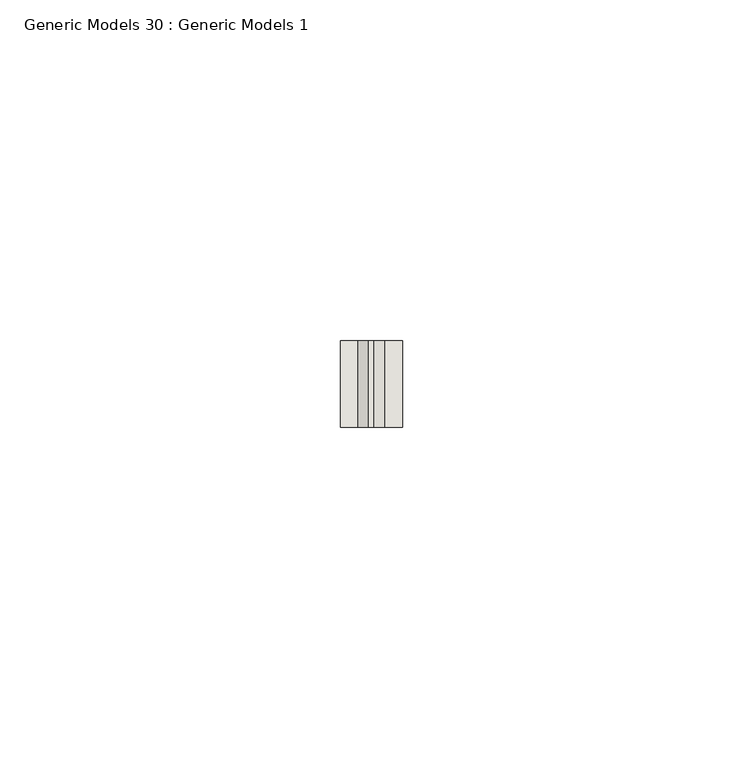
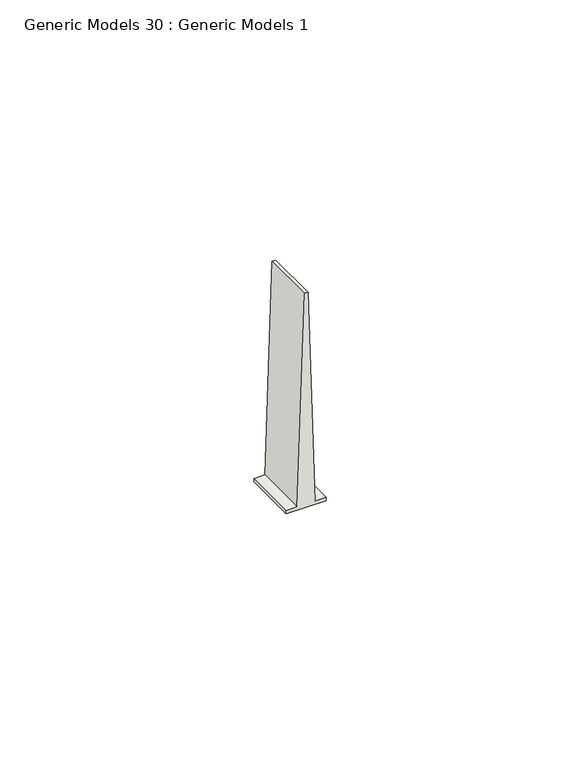
"""IFC4 building model written with IfcOpenShell, lengths in millimetres: wall geometry, Generic Models 30 : Generic Models 1."""

from ifc_helpers import new_model, si_unit, frame, origin, place, context, project, spatial, polyline, outline, extrude, source, transform, mapped, element, save


def generic_models_30_generic_models_1_34d9de7f(model_context):
    return source(origin(), model_context, "Body", "SweptSolid", [
        extrude(outline(polyline([(2455.06875, 49733.4159), (2455.06875, 49742.5091), (2455.8625, 49742.5091), (2455.8625, 49739.9592364), (2506.6625, 49738.3618473), (2506.6625, 49737.5631527), (2455.8625, 49735.9657636), (2455.8625, 49733.4159), (2455.06875, 49733.4159)])), frame((0.0, 565.15, 0.0), z_axis=(0.0, 1.0, 0.0), x_axis=(0.0, 0.0, 1.0)), (0.0, 0.0, 1.0), 12.7),
    ])


if __name__ == "__main__":
    model = new_model("IFC4")
    model_context = context("Model", 3, world=origin())
    ifc_project = project(units=[si_unit("LENGTHUNIT", "METRE", prefix="MILLI")], contexts=[model_context])
    site = spatial("IfcSite", under=ifc_project)
    building = spatial("IfcBuilding", under=site)
    placement = place(None, origin())
    generic_models_30_generic_models_1_shape = generic_models_30_generic_models_1_34d9de7f(model_context)
    element("IfcWall", 1, ObjectType="Generic Models 30 : Generic Models 1", at=placement, inside=building, context=model_context, shape_type="MappedRepresentation", body=[
        mapped(generic_models_30_generic_models_1_shape, transform((0.0, 0.0, 0.0), x_axis=(1.0, 0.0, 0.0), y_axis=(0.0, 1.0, 0.0), z_axis=(0.0, 0.0, 1.0))),
    ])
    save(model, "model.ifc")

# Revit data of these elements
# Element 1 (IfcWall, "Generic Models 30 : Generic Models 1")
#   Materials on its faces: "METAL RUNNER CHANNEL; FASTEN @ 24\" O.C."
# Materials
#   "METAL RUNNER CHANNEL; FASTEN @ 24\" O.C.": class "Unassigned", colour RGB 210 209 208, transparency 0, Keynote = "M05121300.02", Cost = 0
